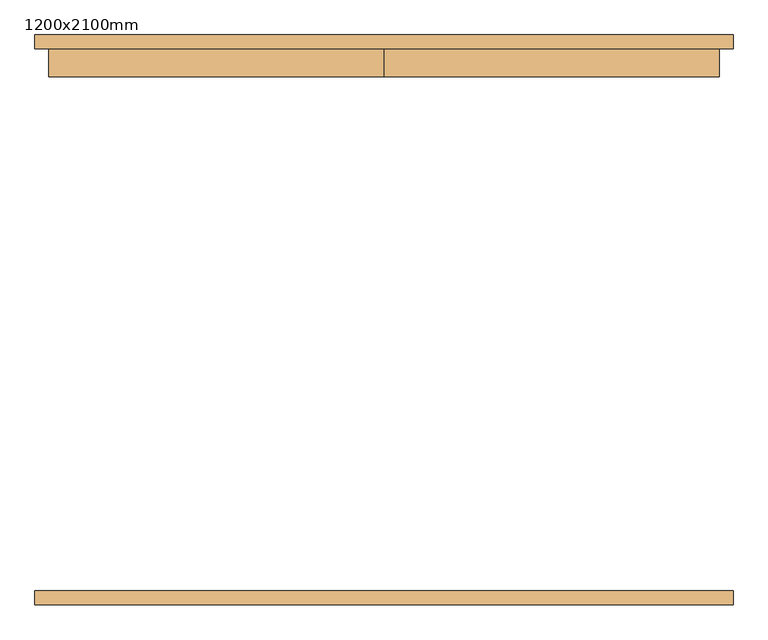
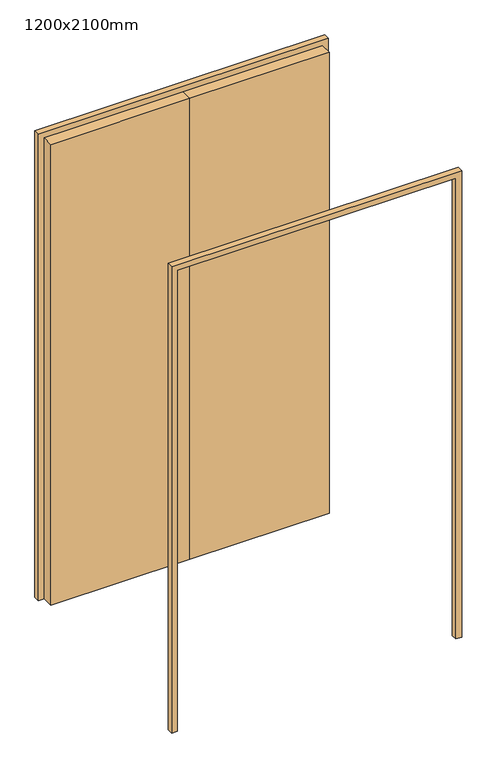
"""IFC4 building model written with IfcOpenShell, lengths in millimetres: door geometry, WWm-DoubleSolid-Flush : 1200x2100mm."""

from ifc_helpers import new_model, si_unit, frame, origin, origin_with_axes, place, context, project, spatial, polyline, outline, extrude, source, transform, mapped, element, save


def door_1200x2100mm_3dafc3e4(model_context):
    return source(origin(), model_context, "Body", "SweptSolid", [
        extrude(outline(polyline([(0.0, 485.0), (600.0, 485.0), (600.0, 435.0), (0.0, 435.0), (0.0, 485.0)])), origin_with_axes(), (0.0, 0.0, 1.0), 2100.0),
        extrude(outline(polyline([(-600.0, 485.0), (0.0, 485.0), (0.0, 435.0), (-600.0, 435.0), (-600.0, 485.0)])), origin_with_axes(), (0.0, 0.0, 1.0), 2100.0),
        extrude(outline(polyline([(2100.0, -600.0), (2100.0, 600.0), (0.0, 600.0), (0.0, 625.0), (2125.0, 625.0), (2125.0, -625.0), (0.0, -625.0), (0.0, -600.0), (2100.0, -600.0)])), frame((0.0, -510.0, 0.0), z_axis=(0.0, 1.0, 0.0), x_axis=(0.0, 0.0, 1.0)), (0.0, 0.0, 1.0), 25.0),
        extrude(outline(polyline([(2100.0, -600.0), (2100.0, 600.0), (0.0, 600.0), (0.0, 625.0), (2125.0, 625.0), (2125.0, -625.0), (0.0, -625.0), (0.0, -600.0), (2100.0, -600.0)])), frame((0.0, 485.0, 0.0), z_axis=(0.0, 1.0, 0.0), x_axis=(0.0, 0.0, 1.0)), (0.0, 0.0, 1.0), 25.0),
    ])


if __name__ == "__main__":
    model = new_model("IFC4")
    model_context = context("Model", 3, world=origin())
    ifc_project = project(units=[si_unit("LENGTHUNIT", "METRE", prefix="MILLI")], contexts=[model_context])
    site = spatial("IfcSite", under=ifc_project)
    building = spatial("IfcBuilding", under=site)
    placement = place(None, origin())
    door_1200x2100mm_shape = door_1200x2100mm_3dafc3e4(model_context)
    element("IfcDoor", 1, ObjectType="WWm-DoubleSolid-Flush : 1200x2100mm", at=placement, inside=building, context=model_context, shape_type="MappedRepresentation", body=[
        mapped(door_1200x2100mm_shape, transform((0.0, 0.0, 0.0), x_axis=(1.0, 0.0, 0.0), y_axis=(0.0, 1.0, 0.0), z_axis=(0.0, 0.0, 1.0))),
    ])
    save(model, "model.ifc")

# Revit data of these elements
# Type "WWm-DoubleSolid-Flush : 1200x2100mm"
#   Type Mark = "EX1-41"
#   Construction Type Id = "MDOOR"
#   Assembly Code = "C1020"
#   Analytic Construction = "Metal"
#   Thickness = 50 mm
#   Thermal Resistance (R) = 0.270117 (m²·K)/W
#   Heat Transfer Coefficient (U) = 3.7021 W/(m²·K)
#   Height = 2100 mm
#   Trim Projection Ext = 25 mm
#   Trim Projection Int = 25 mm
#   Trim Width = 25 mm
#   Width = 1200 mm
#   Not 90 Degree [instance default] = no
#   90 Degree [instance default] = yes
#   Door Material = WW-EC-RGB-White
#   Frame Material = WW-EC-RGB-White
#   Visual Light Transmittance = 0
#   Solar Heat Gain Coefficient = 0
#   Function = (empty or 0)
#   Wall Closure = (empty or 0)
# Element 1 (IfcDoor, "WWm-DoubleSolid-Flush : 1200x2100mm")
#   Materials on its faces: "WW-EC-RGB-White"
# Materials
#   "WW-EC-RGB-White": class "Generic", colour RGB 255 255 255, transparency 0, Comments = "If region requests off-white, swith asset color to RGB 231-228-220", Description = "Generic Color", Cost = 0
